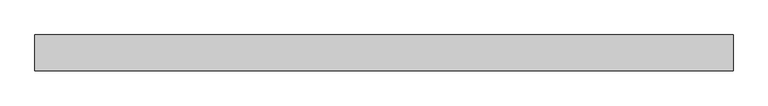
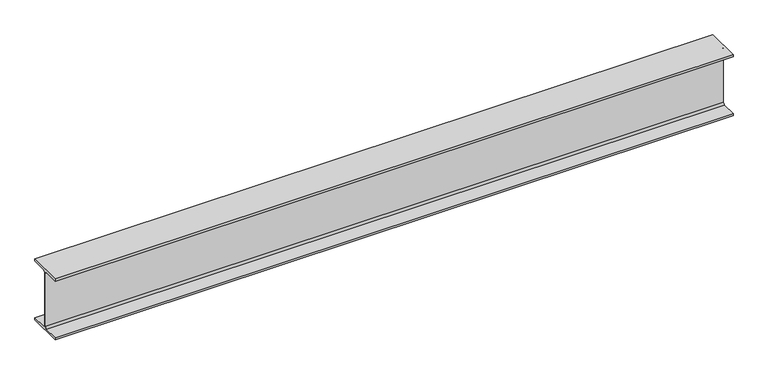
"""IFC4 building model written with IfcOpenShell, lengths in millimetres: beam geometry, Old_Steel Beam_H-KSD3502 : H_SB_ASB_H-200×200x8x12."""

from ifc_helpers import new_model, si_unit, point, frame, frame_2d, origin, place, context, project, spatial, polyline, circle_curve, trimmed, segment, composite_curve, outline, extrude, source, transform, mapped, element, save


def beam_0bb79bd1(model_context):
    return source(origin(), model_context, "Body", "SweptSolid", [
        extrude(outline(composite_curve([segment(polyline([(82.5, -141.5), (82.5, -151.7), (-82.5, -151.7), (-82.5, -141.5), (-11.9, -141.5)]), True, "CONTINUOUS"), segment(trimmed(circle_curve(frame_2d((-11.9, -132.6)), 8.9), [point((-11.9, -141.5))], [point((-3.0, -132.6))], True, "CARTESIAN"), True, "CONTINUOUS"), segment(polyline([(-3.0, -132.6), (-3.0, 132.6)]), True, "CONTINUOUS"), segment(trimmed(circle_curve(frame_2d((-11.9, 132.6)), 8.9), [point((-3.0, 132.6))], [point((-11.9, 141.5))], True, "CARTESIAN"), True, "CONTINUOUS"), segment(polyline([(-11.9, 141.5), (-82.5, 141.5), (-82.5, 151.7), (82.5, 151.7), (82.5, 141.5), (11.9, 141.5)]), True, "CONTINUOUS"), segment(trimmed(circle_curve(frame_2d((11.9, 132.6)), 8.9), [point((11.9, 141.5))], [point((3.0, 132.6))], True, "CARTESIAN"), True, "CONTINUOUS"), segment(polyline([(3.0, 132.6), (3.0, -132.6)]), True, "CONTINUOUS"), segment(trimmed(circle_curve(frame_2d((11.9, -132.6)), 8.9), [point((3.0, -132.6))], [point((11.9, -141.5))], True, "CARTESIAN"), True, "CONTINUOUS"), segment(polyline([(11.9, -141.5), (82.5, -141.5)]), True, "CONTINUOUS")], self_intersect=False)), frame((-1390.503051, 0.0, 0.0), z_axis=(1.0, 0.0, 0.0), x_axis=(0.0, 1.0, 0.0)), (0.0, 0.0, 1.0), 3204.7445716),
    ])


if __name__ == "__main__":
    model = new_model("IFC4")
    model_context = context("Model", 3, world=origin())
    ifc_project = project(units=[si_unit("LENGTHUNIT", "METRE", prefix="MILLI")], contexts=[model_context])
    site = spatial("IfcSite", under=ifc_project)
    building = spatial("IfcBuilding", under=site)
    placement = place(None, origin())
    beam_shape = beam_0bb79bd1(model_context)
    element("IfcBeam", 1, ObjectType="Old_Steel Beam_H-KSD3502 : H_SB_ASB_H-200×200x8x12", at=placement, inside=building, context=model_context, shape_type="MappedRepresentation", body=[
        mapped(beam_shape, transform((0.0, 0.0, 0.0), x_axis=(1.0, 0.0, 0.0), y_axis=(0.0, 1.0, 0.0), z_axis=(0.0, 0.0, 1.0))),
    ])
    save(model, "model.ifc")

# Revit data of these elements
# Type "Old_Steel Beam_H-KSD3502 : H_SB_ASB_H-200×200x8x12"
#   Width = 20.0 cm
#   Web Thickness = 0.8 cm
#   Web Fillet = 1.3 cm
#   Warping Constant = 141376.0 cm⁶
#   Torsional Moment of Inertia = 26.2485 cm⁴
#   Torsional Modulus = 1.0 cm³
#   Section Area = 63.53 cm²
#   Plastic Modulus weak axis = 244.0 cm³
#   Plastic Modulus strong axis = 525.0 cm³
#   Perimeter = 1.16 m²/m
#   Nominal Weight = 49.90 kgf/m
#   Moment of Inertia weak axis = 1600.00 cm⁴
#   Moment of Inertia strong axis = 4720.00 cm⁴
#   Height = 20.0 cm
#   Flange Thickness = 1.2 cm
#   Elastic Modulus weak axis = 160.0 cm³
#   Elastic Modulus strong axis = 472.0 cm³
#   Centroid Vertical = 10.0 cm
#   Centroid Horizontal = 10.0 cm
#   Length [instance default] = 1.5240 m
#   Structural Material [instance default] = Steel, 45-345
#   Assembly Code = ""
# Element 1 (IfcBeam, "Old_Steel Beam_H-KSD3502 : H_SB_ASB_H-200×200x8x12")
#   Structural Material = none
# Materials
#   "Steel, 45-345": class "Metal", colour RGB 189 187 185, transparency 0, Description = "Steel 345 MPa", Cost = 0
